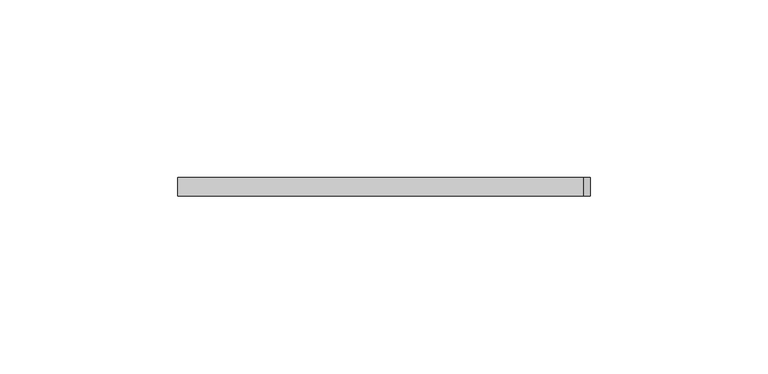
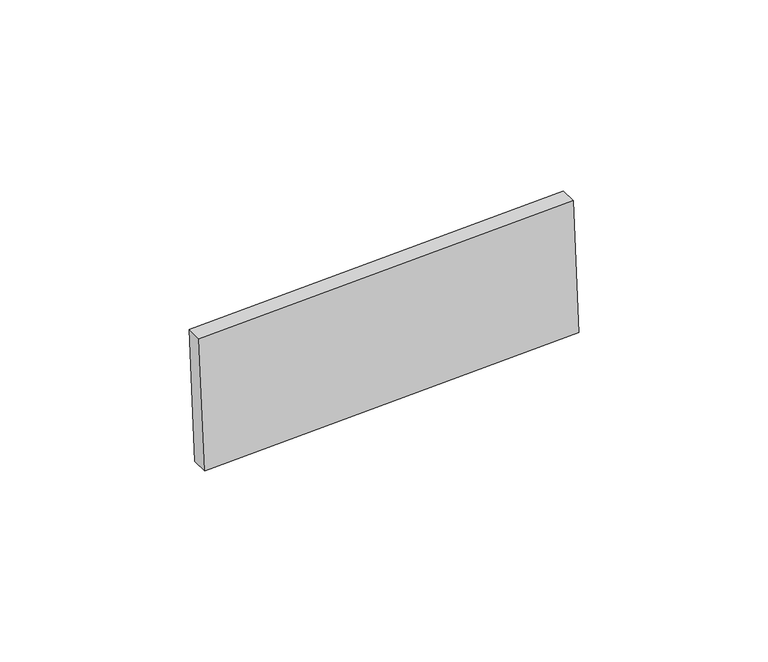
"""IFC4 building model written with IfcOpenShell, lengths in millimetres: proxy geometry, Inner panel:Inner panel:1:Inner panel:1 : Inner panel:Inner panel:300324:2:Inner panel:1:Inner panel:1 : Inner panel:Inner panel:300324:2 : Inner panel:Inner panel:1:Inner panel:1 : Inner panel:Inner panel:300324:300043:146 : Inner panel:Inner panel:1:Inner panel:1 : Inner panel:Inner panel:300324:2:Inner panel:1:Inner panel:1 : Inner panel:Inner panel:300324:2 : Inner panel:Inner panel:1:Inner panel:1 : Inner panel:Inner panel:300324:300043:308120."""

from ifc_helpers import new_model, si_unit, frame, origin, place, context, project, spatial, polyline, outline, extrude, source, transform, mapped, element, save


def generic_models_699962cc(model_context):
    return source(origin(), model_context, "Body", "SweptSolid", [
        extrude(outline(polyline([(0.0, -114.2999999), (0.0, 0.0), (5.2138089, 0.0), (5.2138089, -114.2999999), (0.0, -114.2999999)])), frame((559645.4061496, -578534.9848948, 3922.3662256), z_axis=(-0.04163054471216399, 0.0, 0.9991330730923527), x_axis=(0.0, -1.0, 0.0)), (0.0, 0.0, 1.0), 43.2233908),
    ])


if __name__ == "__main__":
    model = new_model("IFC4")
    model_context = context("Model", 3, world=origin())
    ifc_project = project(units=[si_unit("LENGTHUNIT", "METRE", prefix="MILLI")], contexts=[model_context])
    site = spatial("IfcSite", under=ifc_project)
    building = spatial("IfcBuilding", under=site)
    placement = place(None, origin())
    generic_models_shape = generic_models_699962cc(model_context)
    element("IfcBuildingElementProxy", 1, Name="Inner panel:Inner panel:1:Inner panel:1 : Inner panel:Inner panel:300324:2:Inner panel:1:Inner panel:1 : Inner panel:Inner panel:300324:2 : Inner panel:Inner panel:1:Inner panel:1 : Inner panel:Inner panel:300324:300043:146 : Inner panel:Inner panel:1:Inner panel:1 : Inner panel:Inner panel:300324:2:Inner panel:1:Inner panel:1 : Inner panel:Inner panel:300324:2 : Inner panel:Inner panel:1:Inner panel:1 : Inner panel:Inner panel:300324:300043:308120", ObjectType="Inner panel:Inner panel:1:Inner panel:1 : Inner panel:Inner panel:300324:2:Inner panel:1:Inner panel:1 : Inner panel:Inner panel:300324:2 : Inner panel:Inner panel:1:Inner panel:1 : Inner panel:Inner panel:300324:300043:146 : Inner panel:Inner panel:1:Inner panel:1 : Inner panel:Inner panel:300324:2:Inner panel:1:Inner panel:1 : Inner panel:Inner panel:300324:2 : Inner panel:Inner panel:1:Inner panel:1 : Inner panel:Inner panel:300324:300043:308120", at=placement, inside=building, context=model_context, shape_type="MappedRepresentation", body=[
        mapped(generic_models_shape, transform((0.0, 0.0, 0.0), x_axis=(1.0, 0.0, 0.0), y_axis=(0.0, 1.0, 0.0), z_axis=(0.0, 0.0, 1.0))),
    ])
    save(model, "model.ifc")

# Revit data of these elements
# Type "Inner panel:Inner panel:1:Inner panel:1 : Inner panel:Inner panel:300324:2:Inner panel:1:Inner panel:1 : Inner panel:Inner panel:300324:2 : Inner panel:Inner panel:1:Inner panel:1 : Inner panel:Inner panel:300324:300043:146 : Inner panel:Inner panel:1:Inner panel:1 : Inner panel:Inner panel:300324:2:Inner panel:1:Inner panel:1 : Inner panel:Inner panel:300324:2 : Inner panel:Inner panel:1:Inner panel:1 : Inner panel:Inner panel:300324:300043:308120"
#   NameOverride = "Inner panel:Inner panel:1:Inner panel:1 : Inner panel:Inner panel:300324:2:Inner panel:1:Inner panel:1 : Inner panel:Inner panel:300324:2 : Inner panel:Inner panel:1:Inner panel:1 : Inner panel:Inner panel:300324:300043:308120"
#   ObjectTypeOverride = "Inner panel:1:Inner panel:1 : Inner panel:Inner panel:300324:2 : Inner panel:Inner panel:1:Inner panel:1 : Inner panel:Inner panel:300324:300043"
#   Reference = "Inner panel"
#   Tag = "308120"
# Element 1 (IfcBuildingElementProxy, "Inner panel:Inner panel:1:Inner panel:1 : Inner panel:Inner panel:300324:2:Inner panel:1:Inner panel:1 : Inner panel:Inner panel:300324:2 : Inner panel:Inner panel:1:Inner panel:1 : Inner panel:Inner panel:300324:300043:146 : Inner panel:Inner panel:1:Inner panel:1 : Inner panel:Inner panel:300324:2:Inner panel:1:Inner panel:1 : Inner panel:Inner panel:300324:2 : Inner panel:Inner panel:1:Inner panel:1 : Inner panel:Inner panel:300324:300043:308120")
#   Materials on its faces: "SLIDING CLIP"
# Materials
#   "SLIDING CLIP": class "Generic", colour RGB 120 120 120, transparency 0, Cost = 0
